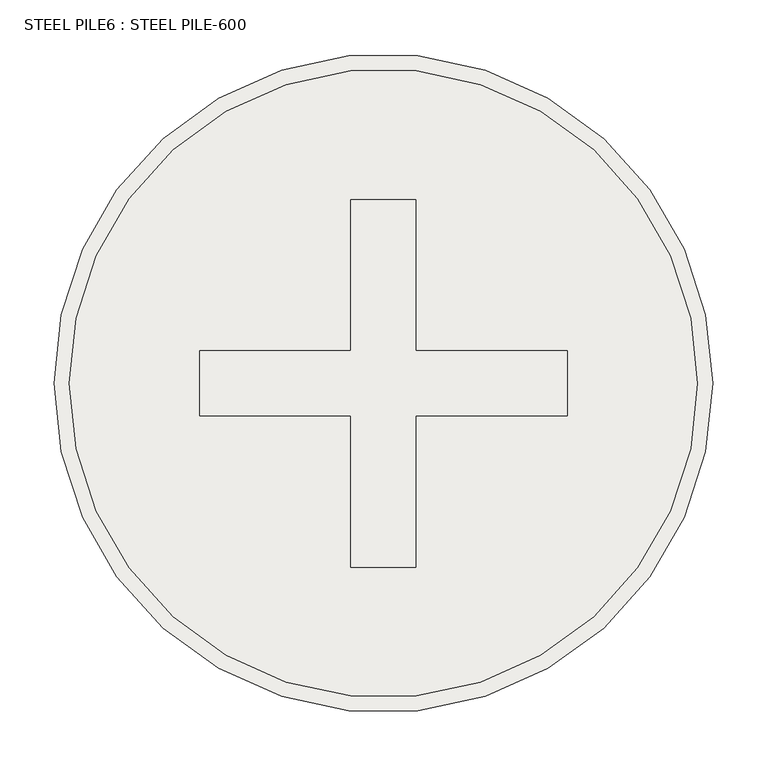
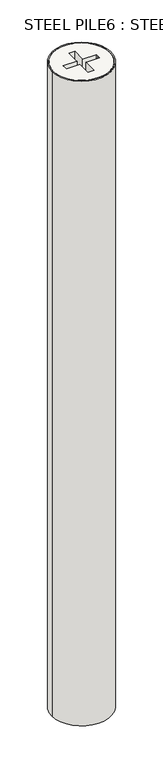
"""IFC4 building model written with IfcOpenShell, lengths in millimetres: slab geometry, STEEL PILE6 : STEEL PILE-600."""

from ifc_helpers import new_model, si_unit, point, frame, frame_2d, origin, place, context, project, spatial, circle_curve, trimmed, segment, composite_curve, outline, extrude, source, transform, mapped, element, save
from ifc_brep_helpers import plane_surface, cylinder_surface, advanced_brep


def steel_pile6_steel_pile_600_8fdb82a6(model_context):
    return source(origin(), model_context, "Body", "SolidModel", [
        advanced_brep(
        [(14709.5, 19499.5208589, 150.0), (15290.5, 19499.5208589, 150.0), (14970.0, 19469.5208589, 150.0), (14830.0, 19469.5208589, 150.0), (14830.0, 19499.5208589, 150.0), (14830.0, 19529.5208589, 150.0), (14970.0, 19529.5208589, 150.0), (14970.0, 19669.5208589, 150.0), (15030.0, 19669.5208589, 150.0), (15030.0, 19529.5208589, 150.0), (15170.0, 19529.5208589, 150.0), (15170.0, 19499.5208589, 150.0), (15170.0, 19469.5208589, 150.0), (15030.0, 19469.5208589, 150.0), (15030.0, 19329.5208589, 150.0), (14970.0, 19329.5208589, 150.0), (14709.5, 19499.5208589, -1850.0), (15290.5, 19499.5208589, -1850.0), (14830.0, 19469.5208589, -160.0), (14970.0, 19469.5208589, -160.0), (14970.0, 19329.5208589, -160.0), (15030.0, 19329.5208589, -160.0), (15030.0, 19469.5208589, -160.0), (15170.0, 19469.5208589, -160.0), (15170.0, 19499.5208589, -160.0), (15170.0, 19529.5208589, -160.0), (15030.0, 19529.5208589, -160.0), (15030.0, 19669.5208589, -160.0), (14970.0, 19669.5208589, -160.0), (14970.0, 19529.5208589, -160.0), (14830.0, 19529.5208589, -160.0), (14830.0, 19499.5208589, -160.0)],
        [
            (0, 1, circle_curve(frame((15000.0, 19499.5208589, 150.0), z_axis=(0.0, 0.0, 1.0), x_axis=(1.0, 0.0, 0.0)), 290.5)),
            (1, 0, circle_curve(frame((15000.0, 19499.5208589, 150.0), z_axis=(0.0, 0.0, 1.0), x_axis=(1.0, 0.0, 0.0)), 290.5)),
            (2, 3),
            (3, 4),
            (4, 5),
            (5, 6),
            (6, 7),
            (7, 8),
            (8, 9),
            (9, 10),
            (10, 11),
            (11, 12),
            (12, 13),
            (13, 14),
            (14, 15),
            (15, 2),
            (16, 17, circle_curve(frame((15000.0, 19499.5208589, -1850.0), z_axis=(0.0, 0.0, -1.0), x_axis=(1.0, 0.0, 0.0)), 290.5)),
            (17, 16, circle_curve(frame((15000.0, 19499.5208589, -1850.0), z_axis=(0.0, 0.0, -1.0), x_axis=(1.0, 0.0, 0.0)), 290.5)),
            (0, 16),
            (17, 1),
            (18, 19),
            (19, 20),
            (20, 21),
            (21, 22),
            (22, 23),
            (23, 24),
            (24, 25),
            (25, 26),
            (26, 27),
            (27, 28),
            (28, 29),
            (29, 30),
            (30, 31),
            (31, 18),
            (18, 3),
            (2, 19),
            (15, 20),
            (14, 21),
            (13, 22),
            (12, 23),
            (11, 24),
            (10, 25),
            (9, 26),
            (8, 27),
            (7, 28),
            (6, 29),
            (5, 30),
            (4, 31),
        ],
        [
            plane_surface(frame((15290.5, 19499.5208589, 150.0), z_axis=(0.0, 0.0, 1.0), x_axis=(0.0, 1.0, 0.0))),
            plane_surface(frame((15290.5, 19499.5208589, -1850.0), z_axis=(0.0, 0.0, -1.0), x_axis=(0.0, -1.0, 0.0))),
            cylinder_surface(frame((15000.0, 19499.5208589, -1850.0), z_axis=(0.0, 0.0, 1.0), x_axis=(1.0, 0.0, 0.0)), 290.5),
            plane_surface(frame((14830.0, 19469.5208589, -160.0), z_axis=(0.0, 0.0, 1.0), x_axis=(-1.0, 0.0, 0.0))),
            plane_surface(frame((14830.0, 19469.5208589, 160.0), z_axis=(0.0, 1.0, 0.0), x_axis=(0.0, 0.0, -1.0))),
            plane_surface(frame((14970.0, 19469.5208589, 160.0), z_axis=(1.0, 0.0, 0.0), x_axis=(0.0, 0.0, -1.0))),
            plane_surface(frame((14970.0, 19329.5208589, 160.0), z_axis=(0.0, 1.0, 0.0), x_axis=(0.0, 0.0, -1.0))),
            plane_surface(frame((15030.0, 19329.5208589, 160.0), z_axis=(-1.0, 0.0, 0.0), x_axis=(0.0, 0.0, -1.0))),
            plane_surface(frame((15030.0, 19469.5208589, 160.0), z_axis=(0.0, 1.0, 0.0), x_axis=(0.0, 0.0, -1.0))),
            plane_surface(frame((15170.0, 19469.5208589, 160.0), z_axis=(-1.0, 0.0, 0.0), x_axis=(0.0, 0.0, -1.0))),
            plane_surface(frame((15170.0, 19499.5208589, 160.0), z_axis=(-1.0, 0.0, 0.0), x_axis=(0.0, 0.0, -1.0))),
            plane_surface(frame((15170.0, 19529.5208589, 160.0), z_axis=(0.0, -1.0, 0.0), x_axis=(0.0, 0.0, -1.0))),
            plane_surface(frame((15030.0, 19529.5208589, 160.0), z_axis=(-1.0, 0.0, 0.0), x_axis=(0.0, 0.0, -1.0))),
            plane_surface(frame((15030.0, 19669.5208589, 160.0), z_axis=(0.0, -1.0, 0.0), x_axis=(0.0, 0.0, -1.0))),
            plane_surface(frame((14970.0, 19669.5208589, 160.0), z_axis=(1.0, 0.0, 0.0), x_axis=(0.0, 0.0, -1.0))),
            plane_surface(frame((14970.0, 19529.5208589, 160.0), z_axis=(0.0, -1.0, 0.0), x_axis=(0.0, 0.0, -1.0))),
            plane_surface(frame((14830.0, 19529.5208589, 160.0), z_axis=(1.0, 0.0, 0.0), x_axis=(0.0, 0.0, -1.0))),
            plane_surface(frame((14830.0, 19499.5208589, 160.0), z_axis=(1.0, 0.0, 0.0), x_axis=(0.0, 0.0, -1.0))),
        ],
        [
            (0, [[1, 2], [3, 4, 5, 6, 7, 8, 9, 10, 11, 12, 13, 14, 15, 16]]),
            (1, [[17, 18]]),
            (2, [[-1, 19, -18, 20]]),
            (2, [[-2, -20, -17, -19]]),
            (3, [[21, 22, 23, 24, 25, 26, 27, 28, 29, 30, 31, 32, 33, 34]]),
            (4, [[-21, 35, -3, 36]]),
            (5, [[-22, -36, -16, 37]]),
            (6, [[-23, -37, -15, 38]]),
            (7, [[-24, -38, -14, 39]]),
            (8, [[-25, -39, -13, 40]]),
            (9, [[-26, -40, -12, 41]]),
            (10, [[-27, -41, -11, 42]]),
            (11, [[-28, -42, -10, 43]]),
            (12, [[-29, -43, -9, 44]]),
            (13, [[-30, -44, -8, 45]]),
            (14, [[-31, -45, -7, 46]]),
            (15, [[-32, -46, -6, 47]]),
            (16, [[-33, -47, -5, 48]]),
            (17, [[-34, -48, -4, -35]]),
        ],
    ),
        extrude(outline(composite_curve([segment(trimmed(circle_curve(frame_2d((15000.0, 19499.5208589)), 304.5), [point((14695.5, 19499.5208589))], [point((15304.5, 19499.5208589))], False, "CARTESIAN"), True, "CONTINUOUS"), segment(trimmed(circle_curve(frame_2d((15000.0, 19499.5208589)), 304.5), [point((15304.5, 19499.5208589))], [point((14695.5, 19499.5208589))], False, "CARTESIAN"), True, "CONTINUOUS")], self_intersect=False), holes=[composite_curve([segment(trimmed(circle_curve(frame_2d((15000.0, 19499.5208589)), 290.5), [point((14709.5, 19499.5208589))], [point((15290.5, 19499.5208589))], True, "CARTESIAN"), True, "CONTINUOUS"), segment(trimmed(circle_curve(frame_2d((15000.0, 19499.5208589)), 290.5), [point((15290.5, 19499.5208589))], [point((14709.5, 19499.5208589))], True, "CARTESIAN"), True, "CONTINUOUS")], self_intersect=False)]), frame((0.0, 0.0, -6850.0), z_axis=(0.0, 0.0, 1.0), x_axis=(1.0, 0.0, 0.0)), (0.0, 0.0, 1.0), 7000.0),
    ])


if __name__ == "__main__":
    model = new_model("IFC4")
    model_context = context("Model", 3, world=origin())
    ifc_project = project(units=[si_unit("LENGTHUNIT", "METRE", prefix="MILLI")], contexts=[model_context])
    site = spatial("IfcSite", under=ifc_project)
    building = spatial("IfcBuilding", under=site)
    placement = place(None, origin())
    steel_pile6_steel_pile_600_shape = steel_pile6_steel_pile_600_8fdb82a6(model_context)
    element("IfcSlab", 1, ObjectType="STEEL PILE6 : STEEL PILE-600", at=placement, inside=building, context=model_context, shape_type="MappedRepresentation", body=[
        mapped(steel_pile6_steel_pile_600_shape, transform((0.0, 0.0, 0.0), x_axis=(1.0, 0.0, 0.0), y_axis=(0.0, 1.0, 0.0), z_axis=(0.0, 0.0, 1.0))),
    ])
    save(model, "model.ifc")
